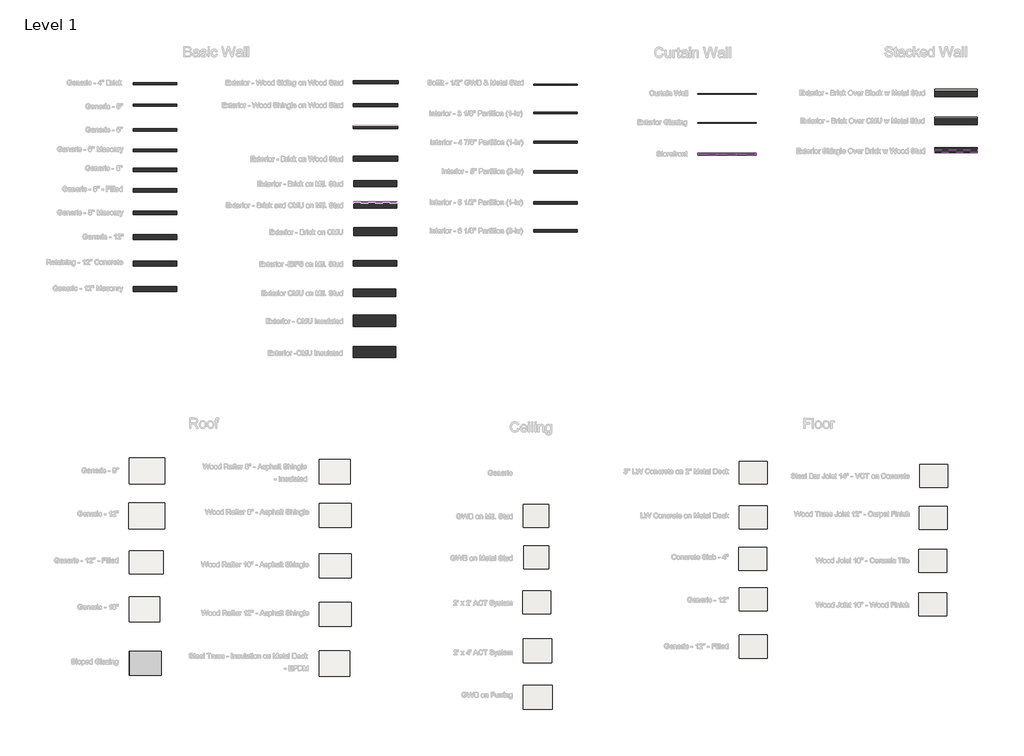
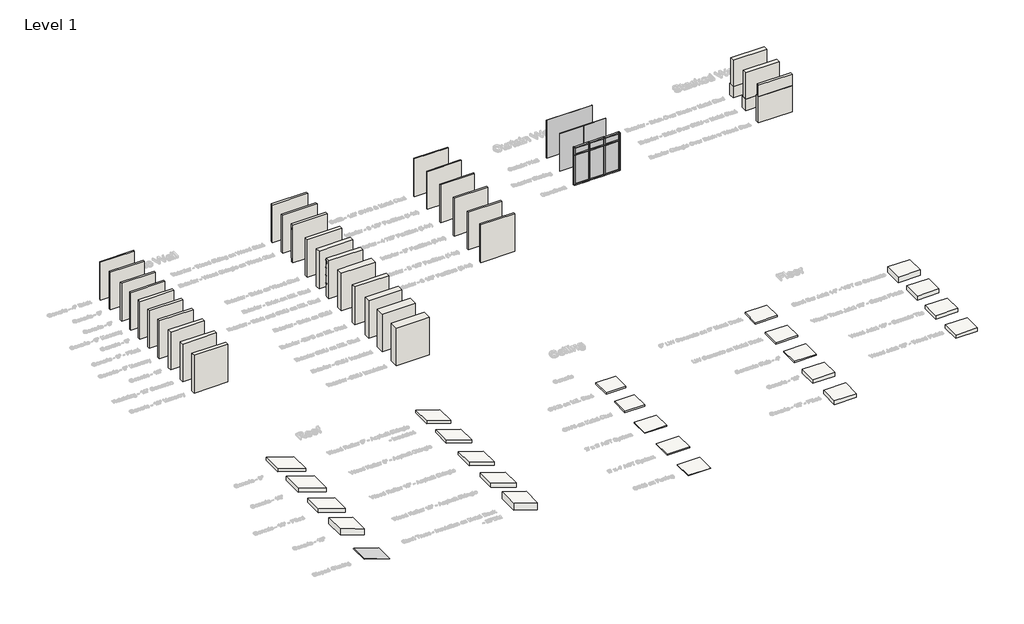
# One storey, part 1 of 42: 33 walls, 17 members, 10 plates, 9 roofs, 9 slabs, 5 coverings, 3 proxies.
"""IFC4 building model written with IfcOpenShell, lengths in millimetres."""

import ifcopenshell
import ifcopenshell.guid

model = None  # the IFC model being written
_history = None  # IfcOwnerHistory: only IFC2X3 demands one
_inside = {}  # id of a spatial element -> (the spatial element, [elements in it])
_under = {}  # id of a project, library or spatial element -> (it, [spatial elements below it])
_declared = {}  # id of a project -> (the project, [libraries it declares])
_typed = {}  # id of a type object -> (the type object, [elements of that type])
_made_of = {}  # id of a material, layer set ... -> (it, [elements and type objects made of it])


def new_model(schema):
    """Start an empty IFC model of exactly this schema.

    Asked for "IFC4X3", IfcOpenShell would pick the latest addendum, in which some entities
    have other attributes; the version numbers below select the first issue.
    IFC2X3 requires an IfcOwnerHistory on every rooted entity: one is made here for all.
    """
    global model, _history
    if schema == "IFC4X3":
        model = ifcopenshell.file(schema_version=(4, 3, 0, 0))
    else:
        model = ifcopenshell.file(schema=schema)
    _inside.clear()
    _under.clear()
    _declared.clear()
    _typed.clear()
    _made_of.clear()
    _history = None
    if model.schema == "IFC2X3":
        org = make("IfcOrganization", Name="unknown")
        user = make(
            "IfcPersonAndOrganization",
            ThePerson=make("IfcPerson", FamilyName="unknown"),
            TheOrganization=org,
        )
        app = make(
            "IfcApplication",
            ApplicationDeveloper=org,
            Version="unknown",
            ApplicationFullName="unknown",
            ApplicationIdentifier="unknown",
        )
        _history = make(
            "IfcOwnerHistory",
            OwningUser=user,
            OwningApplication=app,
            ChangeAction="ADDED",
            CreationDate=0,
        )
    return model


def make(cls, **values):
    """One entity of the class cls with the attributes given. An attribute that is None is left unset."""
    return model.create_entity(
        cls, **{name: value for name, value in values.items() if value is not None}
    )


def rooted(cls, **values):
    """An entity with a GlobalId (a new one), such as an element, a storey or a relation."""
    return make(cls, GlobalId=ifcopenshell.guid.new(), OwnerHistory=_history, **values)


def si_unit(unit_type, name, prefix=None):
    """IfcSIUnit, for example si_unit("LENGTHUNIT", "METRE", prefix="MILLI")."""
    return make("IfcSIUnit", UnitType=unit_type, Prefix=prefix, Name=name)


def assignment(units):
    """IfcUnitAssignment: the units of a project."""
    return None if units is None else make("IfcUnitAssignment", Units=units)


def point(xyz):
    """IfcCartesianPoint."""
    return None if xyz is None else make("IfcCartesianPoint", Coordinates=xyz)


def direction(xyz):
    """IfcDirection."""
    return None if xyz is None else make("IfcDirection", DirectionRatios=xyz)


def frame(location, z_axis=None, x_axis=None):
    """IfcAxis2Placement3D, a coordinate frame: its origin and axes. An axis left out is left unset."""
    return make(
        "IfcAxis2Placement3D",
        Location=point(location),
        Axis=direction(z_axis),
        RefDirection=direction(x_axis),
    )


def origin():
    """The frame at (0, 0, 0) with its axes left unset."""
    return frame((0.0, 0.0, 0.0))


def origin_with_axes():
    """The frame at (0, 0, 0) with the z axis (0, 0, 1) and the x axis (1, 0, 0) written out."""
    return frame((0.0, 0.0, 0.0), z_axis=(0.0, 0.0, 1.0), x_axis=(1.0, 0.0, 0.0))


def place(relative_to, where):
    """IfcLocalPlacement: puts the frame where relative to a parent placement (None: the world)."""
    return make(
        "IfcLocalPlacement", PlacementRelTo=relative_to, RelativePlacement=where
    )


def context(
    kind, dimensions, precision=None, world=None, true_north=None, identifier=None
):
    """IfcGeometricRepresentationContext, for example the 3D "Model" context."""
    return make(
        "IfcGeometricRepresentationContext",
        ContextIdentifier=identifier,
        ContextType=kind,
        CoordinateSpaceDimension=dimensions,
        Precision=precision,
        WorldCoordinateSystem=world,
        TrueNorth=true_north,
    )


def project(units=None, contexts=None):
    """IfcProject with its units and contexts."""
    return rooted(
        "IfcProject",
        Name="project",
        RepresentationContexts=contexts,
        UnitsInContext=assignment(units),
    )


def spatial(cls, under=None, at=None, **own):
    """A site, building, storey or space (cls), placed at a placement, below another one or the project."""
    s = rooted(cls, ObjectPlacement=at, **own)
    if under is not None:
        _under.setdefault(under.id(), (under, []))[1].append(s)
    return s


def polyline(points):
    """IfcPolyline through the points."""
    return make("IfcPolyline", Points=[point(p) for p in points])


def outline(outer, holes=None, kind="AREA"):
    """IfcArbitraryClosedProfileDef: a profile drawn as a closed curve; with holes, ...WithVoids."""
    if holes is None:
        return make("IfcArbitraryClosedProfileDef", ProfileType=kind, OuterCurve=outer)
    return make(
        "IfcArbitraryProfileDefWithVoids",
        ProfileType=kind,
        OuterCurve=outer,
        InnerCurves=holes,
    )


def extrude(swept, where, along, depth):
    """IfcExtrudedAreaSolid: the profile swept, set in the frame where, extruded along a direction by depth."""
    return make(
        "IfcExtrudedAreaSolid",
        SweptArea=swept,
        Position=where,
        ExtrudedDirection=direction(along),
        Depth=depth,
    )


def faces_of(points, faces, orient=None, outer=None):
    """IfcFace entities. A face is a list of loops; a loop is a list of indices into points, from 0.

    orient and outer hold one flag for each loop. By default every Orientation is true, the
    first loop of a face is its IfcFaceOuterBound and the others are IfcFaceBound.
    """
    made = []
    for i, loops in enumerate(faces):
        bounds = []
        for j, loop in enumerate(loops):
            is_outer = j == 0 if outer is None else outer[i][j]
            bounds.append(
                make(
                    "IfcFaceOuterBound" if is_outer else "IfcFaceBound",
                    Bound=make("IfcPolyLoop", Polygon=[points[k] for k in loop]),
                    Orientation=True if orient is None else orient[i][j],
                )
            )
        made.append(make("IfcFace", Bounds=bounds))
    return made


def faceted_brep(points, faces, orient=None, outer=None, voids=None):
    """IfcFacetedBrep: a solid bounded by flat faces; with voids (closed shells), ...WithVoids."""
    shared = [point(p) for p in points]
    hull = make("IfcClosedShell", CfsFaces=faces_of(shared, faces, orient, outer))
    if voids is None:
        return make("IfcFacetedBrep", Outer=hull)
    return make(
        "IfcFacetedBrepWithVoids",
        Outer=hull,
        Voids=[
            make(cls, CfsFaces=faces_of(shared, fs, o, b)) for cls, fs, o, b in voids
        ],
    )


def shape(context_of_items, identifier, shape_type, items):
    """IfcShapeRepresentation: the items that make up one representation, for example the "Body"."""
    return make(
        "IfcShapeRepresentation",
        ContextOfItems=context_of_items,
        RepresentationIdentifier=identifier,
        RepresentationType=shape_type,
        Items=items,
    )


def source(mapping_origin, context_of_items, identifier, shape_type, items):
    """IfcRepresentationMap: a shape defined once, which mapped items show again and again."""
    return make(
        "IfcRepresentationMap",
        MappingOrigin=mapping_origin,
        MappedRepresentation=shape(context_of_items, identifier, shape_type, items),
    )


def transform(
    local_origin,
    x_axis=None,
    y_axis=None,
    z_axis=None,
    scale=None,
    scale2=None,
    scale3=None,
    uniform=True,
):
    """IfcCartesianTransformationOperator3D, or its non-uniform kind. x_axis, y_axis, z_axis: its Axis1, 2, 3."""
    if uniform:
        return make(
            "IfcCartesianTransformationOperator3D",
            Axis1=direction(x_axis),
            Axis2=direction(y_axis),
            LocalOrigin=point(local_origin),
            Scale=scale,
            Axis3=direction(z_axis),
        )
    return make(
        "IfcCartesianTransformationOperator3DnonUniform",
        Axis1=direction(x_axis),
        Axis2=direction(y_axis),
        LocalOrigin=point(local_origin),
        Scale=scale,
        Axis3=direction(z_axis),
        Scale2=scale2,
        Scale3=scale3,
    )


def mapped(mapping_source, mapping_target):
    """IfcMappedItem: shows the shape of a source again, moved by a transform."""
    return make(
        "IfcMappedItem", MappingSource=mapping_source, MappingTarget=mapping_target
    )


def made_of(thing, what):
    """Note that an element or type object is made of a material, layer set ...; save() writes the relation."""
    if what is not None:
        _made_of.setdefault(what.id(), (what, []))[1].append(thing)
    return thing


def element(
    cls,
    number,
    at=None,
    inside=None,
    cuts=None,
    type_object=None,
    material=None,
    context=None,
    identifier="Body",
    shape_type=None,
    held_by="IfcProductDefinitionShape",
    body=None,
    shapes=None,
    **own,
):
    """One element of the class cls, such as IfcWall. Its Tag is "e" and its number.

    at: its placement. inside: the storey or other place that contains it. cuts: it is an
    opening in that element (IfcRelVoidsElement). A single representation is given by context,
    identifier, shape_type and body (its items); several are given by shapes. held_by: the class
    of the entity that holds the representations. save() writes the other relations.
    """
    e = rooted(cls, Tag="e%d" % number, ObjectPlacement=at, **own)
    if body is not None:
        shapes = [shape(context, identifier, shape_type, body)]
    if shapes is not None:
        e.Representation = make(held_by, Representations=shapes)
    if inside is not None:
        _inside.setdefault(inside.id(), (inside, []))[1].append(e)
    if cuts is not None:
        rooted(
            "IfcRelVoidsElement", RelatingBuildingElement=cuts, RelatedOpeningElement=e
        )
    if type_object is not None:
        _typed.setdefault(type_object.id(), (type_object, []))[1].append(e)
    return made_of(e, material)


def aggregate(whole, parts):
    """IfcRelAggregates: a whole, such as a stair, and the parts it consists of."""
    return rooted("IfcRelAggregates", RelatingObject=whole, RelatedObjects=parts)


def save(model, path):
    """Write the relations noted so far, then the file.

    IfcRelAggregates (storeys below a building ...), IfcRelContainedInSpatialStructure (elements
    in a storey), IfcRelDefinesByType, IfcRelAssociatesMaterial and IfcRelDeclares: one each for
    every whole, place, type object, material and project.
    """
    for whole, parts in _under.values():
        aggregate(whole, parts)
    for where, things in _inside.values():
        rooted(
            "IfcRelContainedInSpatialStructure",
            RelatedElements=things,
            RelatingStructure=where,
        )
    for kind, things in _typed.values():
        rooted("IfcRelDefinesByType", RelatedObjects=things, RelatingType=kind)
    for what, things in _made_of.values():
        rooted("IfcRelAssociatesMaterial", RelatedObjects=things, RelatingMaterial=what)
    for by, libraries in _declared.values():
        rooted("IfcRelDeclares", RelatingContext=by, RelatedDefinitions=libraries)
    model.write(path)


def member_f0fea5a5(model_context):
    return source(origin(), model_context, "Body", "SweptSolid", [
        extrude(outline(polyline([(31.75, 63.5), (31.75, -63.5), (-31.75, -63.5), (-31.75, 63.5), (31.75, 63.5)])), frame((0.0, 0.0, -2438.4), z_axis=(0.0, 0.0, 1.0), x_axis=(1.0, 0.0, 0.0)), (0.0, 0.0, 1.0), 2438.4),
    ])


def member_ee409385(model_context):
    return source(origin(), model_context, "Body", "SweptSolid", [
        extrude(outline(polyline([(0.0, 63.5), (0.0, -63.5), (-63.5, -63.5), (-63.5, 63.5), (0.0, 63.5)])), frame((0.0, 0.0, -2438.4), z_axis=(0.0, 0.0, 1.0), x_axis=(1.0, 0.0, 0.0)), (0.0, 0.0, 1.0), 2438.4),
    ])


def member_6e77e263(model_context):
    return source(origin(), model_context, "Body", "SweptSolid", [
        extrude(outline(polyline([(31.75, 63.5), (31.75, -63.5), (-31.75, -63.5), (-31.75, 63.5), (31.75, 63.5)])), frame((0.0, 0.0, -609.6), z_axis=(0.0, 0.0, 1.0), x_axis=(1.0, 0.0, 0.0)), (0.0, 0.0, 1.0), 609.6),
    ])


def member_47bfaf8a(model_context):
    return source(origin(), model_context, "Body", "SweptSolid", [
        extrude(outline(polyline([(0.0, 63.5), (0.0, -63.5), (-63.5, -63.5), (-63.5, 63.5), (0.0, 63.5)])), frame((0.0, 0.0, -609.6), z_axis=(0.0, 0.0, 1.0), x_axis=(1.0, 0.0, 0.0)), (0.0, 0.0, 1.0), 609.6),
    ])


def member_9b1c5889(model_context):
    return source(origin(), model_context, "Body", "SweptSolid", [
        extrude(outline(polyline([(0.0, 63.5), (0.0, -63.5), (-63.5, -63.5), (-63.5, 63.5), (0.0, 63.5)])), frame((0.0, 0.0, -1073.1500001), z_axis=(0.0, 0.0, 1.0), x_axis=(1.0, 0.0, 0.0)), (0.0, 0.0, 1.0), 1073.1500001),
    ])


def member_f5e9651f(model_context):
    return source(origin(), model_context, "Body", "SweptSolid", [
        extrude(outline(polyline([(0.0, 63.5), (0.0, -63.5), (-63.5, -63.5), (-63.5, 63.5), (0.0, 63.5)])), frame((0.0, 0.0, -1104.8999998), z_axis=(0.0, 0.0, 1.0), x_axis=(1.0, 0.0, 0.0)), (0.0, 0.0, 1.0), 1104.8999998),
    ])


def member_0f61b456(model_context):
    return source(origin(), model_context, "Body", "SweptSolid", [
        extrude(outline(polyline([(31.75, 63.5), (31.75, -63.5), (-31.75, -63.5), (-31.75, 63.5), (31.75, 63.5)])), frame((0.0, 0.0, -1073.1500001), z_axis=(0.0, 0.0, 1.0), x_axis=(1.0, 0.0, 0.0)), (0.0, 0.0, 1.0), 1073.1500001),
    ])


def member_766f1680(model_context):
    return source(origin(), model_context, "Body", "SweptSolid", [
        extrude(outline(polyline([(31.75, 63.5), (31.75, -63.5), (-31.75, -63.5), (-31.75, 63.5), (31.75, 63.5)])), frame((0.0, 0.0, -1104.8999998), z_axis=(0.0, 0.0, 1.0), x_axis=(1.0, 0.0, 0.0)), (0.0, 0.0, 1.0), 1104.8999998),
    ])


def system_panel_glazed_bff502fa(model_context):
    return source(origin(), model_context, "Body", "SweptSolid", [
        extrude(outline(polyline([(914.4000002, 19.05), (-914.4000002, 19.05), (-914.4000002, 44.45), (914.4000002, 44.45), (914.4000002, 19.05)])), origin_with_axes(), (0.0, 0.0, 1.0), 3048.0),
    ])


def system_panel_glazed_af99cf8b(model_context):
    return source(origin(), model_context, "Body", "SweptSolid", [
        extrude(outline(polyline([(719.3802866, 19.05), (-719.3802866, 19.05), (-719.3802866, 44.45), (719.3802866, 44.45), (719.3802866, 19.05)])), origin_with_axes(), (0.0, 0.0, 1.0), 2032.8912782),
    ])


def system_panel_glazed_0ae67c42(model_context):
    return source(origin(), model_context, "Body", "SweptSolid", [
        extrude(outline(polyline([(1752.6, 19.05), (-1752.6, 19.05), (-1752.6, 44.45), (1752.6, 44.45), (1752.6, 19.05)])), origin_with_axes(), (0.0, 0.0, 1.0), 3048.0),
    ])


def system_panel_glazed_525848d0(model_context):
    return source(origin(), model_context, "Body", "SweptSolid", [
        extrude(outline(polyline([(838.1999998, 19.05), (-838.1999998, 19.05), (-838.1999998, 44.45), (838.1999998, 44.45), (838.1999998, 19.05)])), origin_with_axes(), (0.0, 0.0, 1.0), 3048.0),
    ])


def system_panel_glazed_2e981f09(model_context):
    return source(origin(), model_context, "Body", "SweptSolid", [
        extrude(outline(polyline([(536.5750001, 19.05), (-536.5750001, 19.05), (-536.5750001, 44.45), (536.5750001, 44.45), (536.5750001, 19.05)])), origin_with_axes(), (0.0, 0.0, 1.0), 2343.15),
    ])


def system_panel_glazed_87980334(model_context):
    return source(origin(), model_context, "Body", "SweptSolid", [
        extrude(outline(polyline([(552.4499999, 19.05), (-552.4499999, 19.05), (-552.4499999, 44.45), (552.4499999, 44.45), (552.4499999, 19.05)])), origin_with_axes(), (0.0, 0.0, 1.0), 2343.15),
    ])


def system_panel_glazed_ed20128f(model_context):
    return source(origin(), model_context, "Body", "SweptSolid", [
        extrude(outline(polyline([(536.5750001, 19.05), (-536.5750001, 19.05), (-536.5750001, 44.45), (536.5750001, 44.45), (536.5750001, 19.05)])), origin_with_axes(), (0.0, 0.0, 1.0), 514.35),
    ])


def system_panel_glazed_d57d3c71(model_context):
    return source(origin(), model_context, "Body", "SweptSolid", [
        extrude(outline(polyline([(552.4499999, 19.05), (-552.4499999, 19.05), (-552.4499999, 44.45), (552.4499999, 44.45), (552.4499999, 19.05)])), origin_with_axes(), (0.0, 0.0, 1.0), 514.35),
    ])


model = new_model("IFC4")

# Units and contexts
model_context = context("Model", 3, world=origin())
ifc_project = project(units=[si_unit("LENGTHUNIT", "METRE", prefix="MILLI")], contexts=[model_context])

# Site, building, storey
site = spatial("IfcSite", under=ifc_project)
building = spatial("IfcBuilding", under=site)
storey = spatial("IfcBuildingStorey", under=building, Name="Level 1", Elevation=0.0)

# Proxies
placement = place(None, origin())
element("IfcBuildingElementProxy", 1, Name="Reveals", at=placement, inside=storey, context=model_context, shape_type="SweptSolid", body=[
    extrude(outline(polyline([(684.9886716, 10254.6257244), (684.9886716, 10346.7007244), (3275.7886716, 10346.7007244), (3275.7886716, 10254.6257244), (684.9886716, 10254.6257244)])), frame((0.0, 0.0, 1625.6), z_axis=(0.0, 0.0, 1.0), x_axis=(1.0, 0.0, 0.0)), (0.0, 0.0, 1.0), 67.7333333),
])
element("IfcBuildingElementProxy", 2, Name="Reveals", at=placement, inside=storey, context=model_context, shape_type="SweptSolid", body=[
    extrude(outline(polyline([(684.9886716, 10254.6257244), (684.9886716, 10346.7007244), (3275.7886716, 10346.7007244), (3275.7886716, 10254.6257244), (684.9886716, 10254.6257244)])), frame((0.0, 0.0, 2235.2), z_axis=(0.0, 0.0, 1.0), x_axis=(1.0, 0.0, 0.0)), (0.0, 0.0, 1.0), 67.7333333),
])
element("IfcBuildingElementProxy", 3, Name="Reveals", at=placement, inside=storey, context=model_context, shape_type="SweptSolid", body=[
    extrude(outline(polyline([(684.9886716, 10254.6257244), (684.9886716, 10346.7007244), (3275.7886716, 10346.7007244), (3275.7886716, 10254.6257244), (684.9886716, 10254.6257244)])), frame((0.0, 0.0, 2844.8), z_axis=(0.0, 0.0, 1.0), x_axis=(1.0, 0.0, 0.0)), (0.0, 0.0, 1.0), 67.7333333),
])

# Coverings
element("IfcCovering", 4, ObjectType="2' x 2' ACT System", at=placement, inside=storey, context=model_context, shape_type="SweptSolid", body=[
    extrude(outline(polyline([(12486.8390819, -13034.2537401), (12486.8390819, -14405.8537401), (10810.4390819, -14405.8537401), (10810.4390819, -13034.2537401), (12486.8390819, -13034.2537401)])), frame((0.0, 0.0, 304.8), z_axis=(0.0, 0.0, 1.0), x_axis=(1.0, 0.0, 0.0)), (0.0, 0.0, 1.0), 57.15),
])
element("IfcCovering", 5, ObjectType="2' x 4' ACT System", at=placement, inside=storey, context=model_context, shape_type="SweptSolid", body=[
    extrude(outline(polyline([(12558.4206915, -15892.7367664), (12558.4206915, -17334.8063753), (10844.136245, -17334.8063753), (10844.136245, -15892.7367664), (12558.4206915, -15892.7367664)])), frame((0.0, 0.0, 304.8), z_axis=(0.0, 0.0, 1.0), x_axis=(1.0, 0.0, 0.0)), (0.0, 0.0, 1.0), 57.15),
])
element("IfcCovering", 6, ObjectType="GWB on Furring", at=placement, inside=storey, context=model_context, shape_type="SweptSolid", body=[
    extrude(outline(polyline([(12572.090991, -18676.3446177), (12572.090991, -20118.4142266), (10857.8065445, -20118.4142266), (10857.8065445, -18676.3446177), (12572.090991, -18676.3446177)])), frame((0.0, 0.0, 304.8), z_axis=(0.0, 0.0, 1.0), x_axis=(1.0, 0.0, 0.0)), (0.0, 0.0, 1.0), 31.75),
])
element("IfcCovering", 7, ObjectType="GWB on Metal Stud", at=placement, inside=storey, context=model_context, shape_type="SweptSolid", body=[
    extrude(outline(polyline([(12388.3840045, -10326.9546667), (12388.3840045, -11698.5546667), (10864.3840045, -11698.5546667), (10864.3840045, -10326.9546667), (12388.3840045, -10326.9546667)])), frame((0.0, 0.0, 304.8), z_axis=(0.0, 0.0, 1.0), x_axis=(1.0, 0.0, 0.0)), (0.0, 0.0, 1.0), 104.775),
])
element("IfcCovering", 8, ObjectType="GWB on Mtl. Stud", at=placement, inside=storey, context=model_context, shape_type="SweptSolid", body=[
    extrude(outline(polyline([(12368.9724668, -7850.547691), (12368.9724668, -9222.147691), (10844.9724668, -9222.147691), (10844.9724668, -7850.547691), (12368.9724668, -7850.547691)])), frame((0.0, 0.0, 304.8), z_axis=(0.0, 0.0, 1.0), x_axis=(1.0, 0.0, 0.0)), (0.0, 0.0, 1.0), 107.95),
])

# Members
member_shape = member_f0fea5a5(model_context)
element("IfcMember", 9, ObjectType="Rectangular Mullion : 2.5\" x 5\" rectangular", at=placement, inside=storey, context=model_context, shape_type="MappedRepresentation", body=[
    mapped(member_shape, transform((22476.9663232, 13175.6086881, 0.0), x_axis=(1.0, 0.0, 0.0), y_axis=(0.0, -1.0, 0.0), z_axis=(0.0, 0.0, -1.0))),
])
element("IfcMember", 10, ObjectType="Rectangular Mullion : 2.5\" x 5\" rectangular", at=placement, inside=storey, context=model_context, shape_type="MappedRepresentation", body=[
    mapped(member_shape, transform((23645.366323, 13175.6086881, 0.0), x_axis=(1.0, 0.0, 0.0), y_axis=(0.0, -1.0, 0.0), z_axis=(0.0, 0.0, -1.0))),
])
member_2_shape = member_ee409385(model_context)
element("IfcMember", 11, ObjectType="Rectangular Mullion : 2.5\" x 5\" rectangular", at=placement, inside=storey, context=model_context, shape_type="MappedRepresentation", body=[
    mapped(member_2_shape, transform((24813.7663231, 13175.6086881, 0.0), x_axis=(1.0, 0.0, 0.0), y_axis=(0.0, -1.0, 0.0), z_axis=(0.0, 0.0, -1.0))),
])
element("IfcMember", 12, ObjectType="Rectangular Mullion : 2.5\" x 5\" rectangular", at=placement, inside=storey, context=model_context, shape_type="MappedRepresentation", body=[
    mapped(member_2_shape, transform((21308.5663231, 13175.6086881, 2438.4), x_axis=(-1.0, 0.0, 0.0), y_axis=(0.0, -1.0, 0.0), z_axis=(0.0, 0.0, 1.0))),
])
member_3_shape = member_6e77e263(model_context)
element("IfcMember", 13, ObjectType="Rectangular Mullion : 2.5\" x 5\" rectangular", at=placement, inside=storey, context=model_context, shape_type="MappedRepresentation", body=[
    mapped(member_3_shape, transform((22476.9663232, 13175.6086881, 2438.4), x_axis=(1.0, 0.0, 0.0), y_axis=(0.0, -1.0, 0.0), z_axis=(0.0, 0.0, -1.0))),
])
element("IfcMember", 14, ObjectType="Rectangular Mullion : 2.5\" x 5\" rectangular", at=placement, inside=storey, context=model_context, shape_type="MappedRepresentation", body=[
    mapped(member_3_shape, transform((23645.366323, 13175.6086881, 2438.4), x_axis=(1.0, 0.0, 0.0), y_axis=(0.0, -1.0, 0.0), z_axis=(0.0, 0.0, -1.0))),
])
member_4_shape = member_47bfaf8a(model_context)
element("IfcMember", 15, ObjectType="Rectangular Mullion : 2.5\" x 5\" rectangular", at=placement, inside=storey, context=model_context, shape_type="MappedRepresentation", body=[
    mapped(member_4_shape, transform((24813.7663231, 13175.6086881, 2438.4), x_axis=(1.0, 0.0, 0.0), y_axis=(0.0, -1.0, 0.0), z_axis=(0.0, 0.0, -1.0))),
])
element("IfcMember", 16, ObjectType="Rectangular Mullion : 2.5\" x 5\" rectangular", at=placement, inside=storey, context=model_context, shape_type="MappedRepresentation", body=[
    mapped(member_4_shape, transform((21308.5663231, 13175.6086881, 3048.0), x_axis=(-1.0, 0.0, 0.0), y_axis=(0.0, -1.0, 0.0), z_axis=(0.0, 0.0, 1.0))),
])
member_5_shape = member_9b1c5889(model_context)
element("IfcMember", 17, ObjectType="Rectangular Mullion : 2.5\" x 5\" rectangular", at=placement, inside=storey, context=model_context, shape_type="MappedRepresentation", body=[
    mapped(member_5_shape, transform((24750.2663231, 13175.6086881, 3048.0), x_axis=(0.0, 0.0, 1.0), y_axis=(0.0, -1.0, 0.0), z_axis=(1.0, 0.0, 0.0))),
])
element("IfcMember", 18, ObjectType="Rectangular Mullion : 2.5\" x 5\" rectangular", at=placement, inside=storey, context=model_context, shape_type="MappedRepresentation", body=[
    mapped(member_5_shape, transform((22445.2163232, 13175.6086881, 3048.0), x_axis=(0.0, 0.0, 1.0), y_axis=(0.0, -1.0, 0.0), z_axis=(1.0, 0.0, 0.0))),
])
element("IfcMember", 19, ObjectType="Rectangular Mullion : 2.5\" x 5\" rectangular", at=placement, inside=storey, context=model_context, shape_type="MappedRepresentation", body=[
    mapped(member_5_shape, transform((21372.0663231, 13175.6086881, 0.0), x_axis=(0.0, 0.0, -1.0), y_axis=(0.0, -1.0, 0.0), z_axis=(-1.0, 0.0, 0.0))),
])
element("IfcMember", 20, ObjectType="Rectangular Mullion : 2.5\" x 5\" rectangular", at=placement, inside=storey, context=model_context, shape_type="MappedRepresentation", body=[
    mapped(member_5_shape, transform((23677.116323, 13175.6086881, 0.0), x_axis=(0.0, 0.0, -1.0), y_axis=(0.0, -1.0, 0.0), z_axis=(-1.0, 0.0, 0.0))),
])
member_6_shape = member_f5e9651f(model_context)
element("IfcMember", 21, ObjectType="Rectangular Mullion : 2.5\" x 5\" rectangular", at=placement, inside=storey, context=model_context, shape_type="MappedRepresentation", body=[
    mapped(member_6_shape, transform((22508.7163232, 13175.6086881, 0.0), x_axis=(0.0, 0.0, -1.0), y_axis=(0.0, -1.0, 0.0), z_axis=(-1.0, 0.0, 0.0))),
])
member_7_shape = member_0f61b456(model_context)
element("IfcMember", 22, ObjectType="Rectangular Mullion : 2.5\" x 5\" rectangular", at=placement, inside=storey, context=model_context, shape_type="MappedRepresentation", body=[
    mapped(member_7_shape, transform((22445.2163232, 13175.6086881, 2438.4), x_axis=(0.0, 0.0, 1.0), y_axis=(0.0, -1.0, 0.0), z_axis=(1.0, 0.0, 0.0))),
])
element("IfcMember", 23, ObjectType="Rectangular Mullion : 2.5\" x 5\" rectangular", at=placement, inside=storey, context=model_context, shape_type="MappedRepresentation", body=[
    mapped(member_7_shape, transform((24750.2663231, 13175.6086881, 2438.4), x_axis=(0.0, 0.0, 1.0), y_axis=(0.0, -1.0, 0.0), z_axis=(1.0, 0.0, 0.0))),
])
member_8_shape = member_766f1680(model_context)
element("IfcMember", 24, ObjectType="Rectangular Mullion : 2.5\" x 5\" rectangular", at=placement, inside=storey, context=model_context, shape_type="MappedRepresentation", body=[
    mapped(member_8_shape, transform((23613.616323, 13175.6086881, 2438.4), x_axis=(0.0, 0.0, 1.0), y_axis=(0.0, -1.0, 0.0), z_axis=(1.0, 0.0, 0.0))),
])
element("IfcMember", 25, ObjectType="Rectangular Mullion : 2.5\" x 5\" rectangular", at=placement, inside=storey, context=model_context, shape_type="MappedRepresentation", body=[
    mapped(member_6_shape, transform((23613.616323, 13175.6086881, 3048.0), x_axis=(0.0, 0.0, 1.0), y_axis=(0.0, -1.0, 0.0), z_axis=(1.0, 0.0, 0.0))),
])

# Plates
system_panel_glazed_shape = system_panel_glazed_bff502fa(model_context)
element("IfcPlate", 26, ObjectType="System Panel : Glazed", at=placement, inside=storey, context=model_context, shape_type="MappedRepresentation", body=[
    mapped(system_panel_glazed_shape, transform((22222.9663232, 15004.4086881, 0.0), x_axis=(1.0, 0.0, 0.0), y_axis=(0.0, 1.0, 0.0), z_axis=(0.0, 0.0, 1.0))),
])
system_panel_glazed_2_shape = system_panel_glazed_af99cf8b(model_context)
element("IfcPlate", 27, ObjectType="System Panel : Glazed", at=placement, inside=storey, context=model_context, shape_type="MappedRepresentation", body=[
    mapped(system_panel_glazed_2_shape, transform((-10836.8268287, -17373.1798963, 0.0), x_axis=(0.0, 1.0, 0.0), y_axis=(-0.3162277660168387, 0.0, -0.9486832980505137), z_axis=(-0.9486832980505137, 0.0, 0.3162277660168387))),
])
system_panel_glazed_3_shape = system_panel_glazed_0ae67c42(model_context)
element("IfcPlate", 28, ObjectType="System Panel : Glazed", at=placement, inside=storey, context=model_context, shape_type="MappedRepresentation", body=[
    mapped(system_panel_glazed_3_shape, transform((23061.1663231, 16757.0086881, 0.0), x_axis=(1.0, 0.0, 0.0), y_axis=(0.0, 1.0, 0.0), z_axis=(0.0, 0.0, 1.0))),
])
system_panel_glazed_4_shape = system_panel_glazed_525848d0(model_context)
element("IfcPlate", 29, ObjectType="System Panel : Glazed", at=placement, inside=storey, context=model_context, shape_type="MappedRepresentation", body=[
    mapped(system_panel_glazed_4_shape, transform((23975.5663232, 15004.4086881, 0.0), x_axis=(1.0, 0.0, 0.0), y_axis=(0.0, 1.0, 0.0), z_axis=(0.0, 0.0, 1.0))),
])
system_panel_glazed_5_shape = system_panel_glazed_2e981f09(model_context)
element("IfcPlate", 30, ObjectType="System Panel : Glazed", at=placement, inside=storey, context=model_context, shape_type="MappedRepresentation", body=[
    mapped(system_panel_glazed_5_shape, transform((21908.6413231, 13175.6086881, 63.5), x_axis=(1.0, 0.0, 0.0), y_axis=(0.0, 1.0, 0.0), z_axis=(0.0, 0.0, 1.0))),
])
element("IfcPlate", 31, ObjectType="System Panel : Glazed", at=placement, inside=storey, context=model_context, shape_type="MappedRepresentation", body=[
    mapped(system_panel_glazed_5_shape, transform((24213.691323, 13175.6086881, 63.5), x_axis=(1.0, 0.0, 0.0), y_axis=(0.0, 1.0, 0.0), z_axis=(0.0, 0.0, 1.0))),
])
system_panel_glazed_6_shape = system_panel_glazed_87980334(model_context)
element("IfcPlate", 32, ObjectType="System Panel : Glazed", at=placement, inside=storey, context=model_context, shape_type="MappedRepresentation", body=[
    mapped(system_panel_glazed_6_shape, transform((23061.1663231, 13175.6086881, 63.5), x_axis=(1.0, 0.0, 0.0), y_axis=(0.0, 1.0, 0.0), z_axis=(0.0, 0.0, 1.0))),
])
system_panel_glazed_7_shape = system_panel_glazed_ed20128f(model_context)
element("IfcPlate", 33, ObjectType="System Panel : Glazed", at=placement, inside=storey, context=model_context, shape_type="MappedRepresentation", body=[
    mapped(system_panel_glazed_7_shape, transform((21908.6413231, 13175.6086881, 2470.15), x_axis=(1.0, 0.0, 0.0), y_axis=(0.0, 1.0, 0.0), z_axis=(0.0, 0.0, 1.0))),
])
element("IfcPlate", 34, ObjectType="System Panel : Glazed", at=placement, inside=storey, context=model_context, shape_type="MappedRepresentation", body=[
    mapped(system_panel_glazed_7_shape, transform((24213.691323, 13175.6086881, 2470.15), x_axis=(1.0, 0.0, 0.0), y_axis=(0.0, 1.0, 0.0), z_axis=(0.0, 0.0, 1.0))),
])
system_panel_glazed_8_shape = system_panel_glazed_d57d3c71(model_context)
element("IfcPlate", 35, ObjectType="System Panel : Glazed", at=placement, inside=storey, context=model_context, shape_type="MappedRepresentation", body=[
    mapped(system_panel_glazed_8_shape, transform((23061.1663231, 13175.6086881, 2470.15), x_axis=(1.0, 0.0, 0.0), y_axis=(0.0, 1.0, 0.0), z_axis=(0.0, 0.0, 1.0))),
])

# Roofs
element("IfcRoof", 36, ObjectType="Generic - 12\"", at=placement, inside=storey, context=model_context, shape_type="SweptSolid", body=[
    extrude(outline(polyline([(321.2874103, -10641.6185973), (1036.789438, -12788.1246804), (715.5020277, -12788.1246804), (0.0, -10641.6185973), (321.2874103, -10641.6185973)])), frame((0.0, -9316.4021182, 0.0), z_axis=(0.0, 1.0, 0.0), x_axis=(0.0, 0.0, 1.0)), (0.0, 0.0, 1.0), 1579.5625),
])
element("IfcRoof", 37, ObjectType="Generic - 12\" - Filled", at=placement, inside=storey, context=model_context, shape_type="SweptSolid", body=[
    extrude(outline(polyline([(321.2874103, -10734.0001224), (1003.1050879, -12779.4531552), (681.8176776, -12779.4531552), (0.0, -10734.0001224), (321.2874103, -10734.0001224)])), frame((0.0, -12001.3744682, 0.0), z_axis=(0.0, 1.0, 0.0), x_axis=(0.0, 0.0, 1.0)), (0.0, 0.0, 1.0), 1383.6280937),
])
element("IfcRoof", 38, ObjectType="Generic - 18\"", at=placement, inside=storey, context=model_context, shape_type="SweptSolid", body=[
    extrude(outline(polyline([(481.9311154, -10928.8051732), (1098.8137761, -12779.4531552), (616.8826607, -12779.4531552), (0.0, -10928.8051732), (481.9311154, -10928.8051732)])), frame((0.0, -14869.9869682, 0.0), z_axis=(0.0, 1.0, 0.0), x_axis=(0.0, 0.0, 1.0)), (0.0, 0.0, 1.0), 1497.2020884),
])
element("IfcRoof", 39, ObjectType="Generic - 9\"", at=placement, inside=storey, context=model_context, shape_type="SweptSolid", body=[
    extrude(outline(polyline([(240.9655577, -10645.8531552), (952.1655577, -12779.4531552), (711.2, -12779.4531552), (0.0, -10645.8531552), (240.9655577, -10645.8531552)])), frame((0.0, -6597.0146182, 0.0), z_axis=(0.0, 1.0, 0.0), x_axis=(0.0, 0.0, 1.0)), (0.0, 0.0, 1.0), 1534.3628563),
])
element("IfcRoof", 40, ObjectType="Steel Truss - Insulation on Metal Deck - EPDM", at=placement, inside=storey, context=model_context, shape_type="SweptSolid", body=[
    extrude(outline(polyline([(575.6399434, 451.8559594), (1185.2399434, -1376.9440406), (609.6, -1376.9440406), (0.0, 451.8559594), (575.6399434, 451.8559594)])), frame((0.0, -18138.4509823, 0.0), z_axis=(0.0, 1.0, 0.0), x_axis=(0.0, 0.0, 1.0)), (0.0, 0.0, 1.0), 1524.0),
])
element("IfcRoof", 41, ObjectType="Wood Rafter 10\" - Asphalt Shingle", at=placement, inside=storey, context=model_context, shape_type="SweptSolid", body=[
    extrude(outline(polyline([(274.4329963, 542.7798174), (917.2896637, -1385.790185), (642.8566675, -1385.790185), (0.0, 542.7798174), (274.4329963, 542.7798174)])), frame((0.0, -12251.6321179, 0.0), z_axis=(0.0, 1.0, 0.0), x_axis=(0.0, 0.0, 1.0)), (0.0, 0.0, 1.0), 1438.7605731),
])
element("IfcRoof", 42, ObjectType="Wood Rafter 12\" - Asphalt Shingle", at=placement, inside=storey, context=model_context, shape_type="SweptSolid", body=[
    extrude(outline(polyline([(327.980898, 542.7798174), (970.8375654, -1385.790185), (642.8566675, -1385.790185), (0.0, 542.7798174), (327.980898, 542.7798174)])), frame((0.0, -15148.992691, 0.0), z_axis=(0.0, 1.0, 0.0), x_axis=(0.0, 0.0, 1.0)), (0.0, 0.0, 1.0), 1438.7605731),
])
element("IfcRoof", 43, ObjectType="Wood Rafter 8\" - Asphalt Shingle", at=placement, inside=storey, context=model_context, shape_type="SweptSolid", body=[
    extrude(outline(polyline([(220.8850946, 545.7910112), (863.741762, -1382.7789912), (642.8566675, -1382.7789912), (0.0, 545.7910112), (220.8850946, 545.7910112)])), frame((0.0, -9229.8693805, 0.0), z_axis=(0.0, 1.0, 0.0), x_axis=(0.0, 0.0, 1.0)), (0.0, 0.0, 1.0), 1438.7605731),
])
element("IfcRoof", 44, ObjectType="Wood Rafter 8\" - Asphalt Shingle - Insulated", at=placement, inside=storey, context=model_context, shape_type="SweptSolid", body=[
    extrude(outline(polyline([(224.2318384, 475.5814538), (841.1144991, -1375.0665283), (616.8826607, -1375.0665283), (0.0, 475.5814538), (224.2318384, 475.5814538)])), frame((0.0, -6594.6223043, 0.0), z_axis=(0.0, 1.0, 0.0), x_axis=(0.0, 0.0, 1.0)), (0.0, 0.0, 1.0), 1445.5405937),
])

# Slabs
element("IfcSlab", 45, ObjectType="Wood Truss  Joist 12\" - Carpet Finish ", at=placement, inside=storey, context=model_context, shape_type="SweptSolid", body=[
    extrude(outline(polyline([(36266.767036, -7964.1153855), (36266.767036, -9335.7153855), (34590.367036, -9335.7153855), (34590.367036, -7964.1153855), (36266.767036, -7964.1153855)])), frame((0.0, 0.0, -323.85), z_axis=(0.0, 0.0, 1.0), x_axis=(1.0, 0.0, 0.0)), (0.0, 0.0, 1.0), 323.85),
])
element("IfcSlab", 46, ObjectType="3\" LW Concrete on 2\" Metal Deck", at=placement, inside=storey, context=model_context, shape_type="SweptSolid", body=[
    extrude(outline(polyline([(25462.297259, -5250.8171932), (25462.297259, -6622.4171932), (23785.897259, -6622.4171932), (23785.897259, -5250.8171932), (25462.297259, -5250.8171932)])), frame((0.0, 0.0, -127.0), z_axis=(0.0, 0.0, 1.0), x_axis=(1.0, 0.0, 0.0)), (0.0, 0.0, 1.0), 127.0),
])
element("IfcSlab", 47, ObjectType="Concrete Slab - 4\"", at=placement, inside=storey, context=model_context, shape_type="SweptSolid", body=[
    extrude(outline(polyline([(25449.5750317, -10417.8079652), (25449.5750317, -11789.4079652), (23773.1750317, -11789.4079652), (23773.1750317, -10417.8079652), (25449.5750317, -10417.8079652)])), frame((0.0, 0.0, -101.6), z_axis=(0.0, 0.0, 1.0), x_axis=(1.0, 0.0, 0.0)), (0.0, 0.0, 1.0), 101.6),
])
element("IfcSlab", 48, ObjectType="Generic - 12\"", at=placement, inside=storey, context=model_context, shape_type="SweptSolid", body=[
    extrude(outline(polyline([(25457.124359, -12846.3368689), (25457.124359, -14217.9368689), (23780.724359, -14217.9368689), (23780.724359, -12846.3368689), (25457.124359, -12846.3368689)])), frame((0.0, 0.0, -304.8), z_axis=(0.0, 0.0, 1.0), x_axis=(1.0, 0.0, 0.0)), (0.0, 0.0, 1.0), 304.8),
])
element("IfcSlab", 49, ObjectType="Generic - 12\" - Filled", at=placement, inside=storey, context=model_context, shape_type="SweptSolid", body=[
    extrude(outline(polyline([(25473.8528339, -15648.3022704), (25473.8528339, -17070.7022704), (23797.4528339, -17070.7022704), (23797.4528339, -15648.3022704), (25473.8528339, -15648.3022704)])), frame((0.0, 0.0, -304.8), z_axis=(0.0, 0.0, 1.0), x_axis=(1.0, 0.0, 0.0)), (0.0, 0.0, 1.0), 304.8),
])
element("IfcSlab", 50, ObjectType="LW Concrete on Metal Deck", at=placement, inside=storey, context=model_context, shape_type="SweptSolid", body=[
    extrude(outline(polyline([(25464.6636445, -7938.3779014), (25464.6636445, -9309.9779014), (23788.2636445, -9309.9779014), (23788.2636445, -7938.3779014), (25464.6636445, -7938.3779014)])), frame((0.0, 0.0, -104.775), z_axis=(0.0, 0.0, 1.0), x_axis=(1.0, 0.0, 0.0)), (0.0, 0.0, 1.0), 104.775),
])
element("IfcSlab", 51, ObjectType="Steel Bar Joist 14\" - VCT on Concrete", at=placement, inside=storey, context=model_context, shape_type="SweptSolid", body=[
    extrude(outline(polyline([(36284.0122585, -5434.5515682), (36284.0122585, -6806.1515682), (34607.6122585, -6806.1515682), (34607.6122585, -5434.5515682), (36284.0122585, -5434.5515682)])), frame((0.0, 0.0, -441.325), z_axis=(0.0, 0.0, 1.0), x_axis=(1.0, 0.0, 0.0)), (0.0, 0.0, 1.0), 441.325),
])
element("IfcSlab", 52, ObjectType="Wood Joist 10\" - Ceramic Tile", at=placement, inside=storey, context=model_context, shape_type="SweptSolid", body=[
    extrude(outline(polyline([(36216.4995459, -10528.7510967), (36216.4995459, -11900.3510967), (34540.0995459, -11900.3510967), (34540.0995459, -10528.7510967), (36216.4995459, -10528.7510967)])), frame((0.0, 0.0, -273.05), z_axis=(0.0, 0.0, 1.0), x_axis=(1.0, 0.0, 0.0)), (0.0, 0.0, 1.0), 273.05),
])
element("IfcSlab", 53, ObjectType="Wood Joist 10\" - Wood Finish", at=placement, inside=storey, context=model_context, shape_type="SweptSolid", body=[
    extrude(outline(polyline([(36231.4850833, -13137.5746207), (36231.4850833, -14509.1746207), (34555.0850833, -14509.1746207), (34555.0850833, -13137.5746207), (36231.4850833, -13137.5746207)])), frame((0.0, 0.0, -273.05), z_axis=(0.0, 0.0, 1.0), x_axis=(1.0, 0.0, 0.0)), (0.0, 0.0, 1.0), 273.05),
])

# Walls
element("IfcWall", 54, ObjectType="Soffit - 1/2\" GWB & Metal Stud", at=placement, inside=storey, context=model_context, shape_type="SweptSolid", body=[
    extrude(outline(polyline([(14079.2439264, 17311.8960361), (11488.4439264, 17311.8960361), (11488.4439264, 17362.6960361), (14079.2439264, 17362.6960361), (14079.2439264, 17311.8960361)])), origin_with_axes(), (0.0, 0.0, 1.0), 3048.0),
])
element("IfcWall", 55, ObjectType="Exterior - Wood Shingle over Wood Siding on Wood Stud", at=placement, inside=storey, context=model_context, shape_type="Brep", body=[
    faceted_brep([(668.8686716, 14685.8878373, 0.0), (3310.4686716, 14685.8878373, 0.0), (3310.4686716, 14685.8878373, 3048.0), (668.8686716, 14685.8878373, 3048.0), (668.8686716, 14873.2128373, 0.0), (668.8686716, 14873.2128373, 254.0), (668.8686716, 14873.2128373, 2559.05), (668.8686716, 14873.2128373, 2743.2), (668.8686716, 14873.2128373, 3048.0), (3310.4686716, 14873.2128373, 3048.0), (3310.4686716, 14873.2128373, 2743.2), (3310.4686716, 14873.2128373, 2559.05), (3310.4686716, 14873.2128373, 254.0), (3310.4686716, 14873.2128373, 0.0)], [[[0, 1, 2, 3]], [[4, 5, 6, 7, 8, 9, 10, 11, 12, 13]], [[1, 0, 4, 13]], [[2, 1, 13, 12, 11, 10, 9]], [[3, 2, 9, 8]], [[0, 3, 8, 7, 6, 5, 4]]]),
])
element("IfcWall", 56, ObjectType="Exterior - Block on Mtl. Stud", at=placement, inside=storey, context=model_context, shape_type="Brep", body=[
    faceted_brep([(35496.1518113, 16604.091373, 0.0), (38067.522891, 16604.091373, 0.0), (38067.522891, 16604.091373, 900.0), (35496.1518113, 16604.091373, 900.0), (35496.1518113, 17064.091373, 0.0), (35496.1518113, 17064.091373, 900.0), (38067.522891, 17064.091373, 900.0), (38067.522891, 17064.091373, 0.0), (38067.522891, 16956.616373, 900.0), (35496.1518113, 16956.616373, 900.0)], [[[0, 1, 2, 3]], [[4, 5, 6, 7]], [[1, 0, 4, 7]], [[2, 1, 7, 6, 8]], [[3, 2, 8, 6, 5, 9]], [[0, 3, 9, 5, 4]]]),
])
element("IfcWall", 57, ObjectType="Exterior - Brick and CMU on MTL. Stud", at=placement, inside=storey, context=model_context, shape_type="SweptSolid", body=[
    extrude(outline(polyline([(9927.6007244, 0.0), (9927.6007244, 3048.0), (10280.0257244, 3048.0), (10280.0257244, 2912.5333333), (10254.6257244, 2912.5333333), (10254.6257244, 2844.8), (10187.9507244, 2844.8), (10187.9507244, 2641.6), (10280.0257244, 2641.6), (10280.0257244, 2302.9333333), (10254.6257244, 2302.9333333), (10254.6257244, 2235.2), (10280.0257244, 2235.2), (10280.0257244, 1693.3333333), (10254.6257244, 1693.3333333), (10254.6257244, 1625.6), (10280.0257244, 1625.6), (10280.0257244, 1085.85), (10187.9507244, 1085.85), (10187.9507244, 1016.0), (10280.0257244, 1016.0), (10280.0257244, 0.0), (10187.9507244, 0.0), (9927.6007244, 0.0)])), frame((684.9886716, 0.0, 0.0), z_axis=(1.0, 0.0, 0.0), x_axis=(0.0, 1.0, 0.0)), (0.0, 0.0, 1.0), 2590.8),
])
element("IfcWall", 58, ObjectType="Exterior - Brick on CMU", at=placement, inside=storey, context=model_context, shape_type="SweptSolid", body=[
    extrude(outline(polyline([(3275.7886716, 8281.3632244), (684.9886716, 8281.3632244), (684.9886716, 8776.6632244), (3275.7886716, 8776.6632244), (3275.7886716, 8281.3632244)])), origin_with_axes(), (0.0, 0.0, 1.0), 3048.0),
])
element("IfcWall", 59, ObjectType="Exterior - Brick on Mtl. Stud", at=placement, inside=storey, context=model_context, shape_type="SweptSolid", body=[
    extrude(outline(polyline([(3275.7886716, 11223.0007244), (684.9886716, 11223.0007244), (684.9886716, 11575.4257244), (3275.7886716, 11575.4257244), (3275.7886716, 11223.0007244)])), origin_with_axes(), (0.0, 0.0, 1.0), 3048.0),
])
element("IfcWall", 60, ObjectType="Exterior - Brick on Mtl. Stud", at=placement, inside=storey, context=model_context, shape_type="SweptSolid", body=[
    extrude(outline(polyline([(38067.522891, 16604.191373), (35496.1518113, 16604.191373), (35496.1518113, 16956.616373), (38067.522891, 16956.616373), (38067.522891, 16604.191373)])), frame((0.0, 0.0, 900.0), z_axis=(0.0, 0.0, 1.0), x_axis=(1.0, 0.0, 0.0)), (0.0, 0.0, 1.0), 2148.0),
])
element("IfcWall", 61, ObjectType="Exterior - Brick on Mtl. Stud", at=placement, inside=storey, context=model_context, shape_type="SweptSolid", body=[
    extrude(outline(polyline([(38067.522891, 14930.678873), (35496.1518113, 14930.678873), (35496.1518113, 15283.103873), (38067.522891, 15283.103873), (38067.522891, 14930.678873)])), frame((0.0, 0.0, 914.4), z_axis=(0.0, 0.0, 1.0), x_axis=(1.0, 0.0, 0.0)), (0.0, 0.0, 1.0), 2133.6),
])
element("IfcWall", 62, ObjectType="Exterior - Brick on Wood Stud", at=placement, inside=storey, context=model_context, shape_type="SweptSolid", body=[
    extrude(outline(polyline([(3310.4686716, 12758.6628373), (668.8686716, 12758.6628373), (668.8686716, 13041.2378373), (3310.4686716, 13041.2378373), (3310.4686716, 12758.6628373)])), origin_with_axes(), (0.0, 0.0, 1.0), 3048.0),
])
element("IfcWall", 63, ObjectType="Exterior - Brick on Wood Stud", at=placement, inside=storey, context=model_context, shape_type="Brep", body=[
    faceted_brep([(35496.1518113, 13263.803873, 0.0), (38067.522891, 13263.803873, 0.0), (38067.522891, 13263.803873, 2133.6), (35496.1518113, 13263.803873, 2133.6), (35496.1518113, 13546.378873, 0.0), (35496.1518113, 13546.378873, 2133.6), (38067.522891, 13546.378873, 2133.6), (38067.522891, 13546.378873, 0.0), (38067.522891, 13444.778873, 2133.6), (35496.1518113, 13444.778873, 2133.6)], [[[0, 1, 2, 3]], [[4, 5, 6, 7]], [[1, 0, 4, 7]], [[2, 1, 7, 6, 8]], [[3, 2, 8, 6, 5, 9]], [[0, 3, 9, 5, 4]]]),
])
element("IfcWall", 64, ObjectType="Exterior - CMU Insulated", at=placement, inside=storey, context=model_context, shape_type="SweptSolid", body=[
    extrude(outline(polyline([(3205.5597513, 958.2654873), (668.8686716, 958.2654873), (668.8686716, 1631.3654873), (3205.5597513, 1631.3654873), (3205.5597513, 958.2654873)])), origin_with_axes(), (0.0, 0.0, 1.0), 3048.0),
])
element("IfcWall", 65, ObjectType="Exterior - CMU Insulated", at=placement, inside=storey, context=model_context, shape_type="SweptSolid", body=[
    extrude(outline(polyline([(3205.5597513, 2838.5798121), (668.8686716, 2838.5798121), (668.8686716, 3511.6798121), (3205.5597513, 3511.6798121), (3205.5597513, 2838.5798121)])), origin_with_axes(), (0.0, 0.0, 1.0), 3048.0),
])
element("IfcWall", 66, ObjectType="Exterior - CMU on Mtl. Stud", at=placement, inside=storey, context=model_context, shape_type="SweptSolid", body=[
    extrude(outline(polyline([(3205.5597513, 4623.8029873), (668.8686716, 4623.8029873), (668.8686716, 5077.8279873), (3205.5597513, 5077.8279873), (3205.5597513, 4623.8029873)])), origin_with_axes(), (0.0, 0.0, 1.0), 3048.0),
])
element("IfcWall", 67, ObjectType="Exterior - CMU on Mtl. Stud", at=placement, inside=storey, context=model_context, shape_type="Brep", body=[
    faceted_brep([(35496.1518113, 14930.678873, 0.0), (38067.522891, 14930.678873, 0.0), (38067.522891, 14930.678873, 914.4), (35496.1518113, 14930.678873, 914.4), (35496.1518113, 15384.703873, 0.0), (35496.1518113, 15384.703873, 914.4), (38067.522891, 15384.703873, 914.4), (38067.522891, 15384.703873, 0.0), (38067.522891, 15283.103873, 914.4), (35496.1518113, 15283.103873, 914.4)], [[[0, 1, 2, 3]], [[4, 5, 6, 7]], [[1, 0, 4, 7]], [[2, 1, 7, 6, 8]], [[3, 2, 8, 6, 5, 9]], [[0, 3, 9, 5, 4]]]),
])
element("IfcWall", 68, ObjectType="Exterior - EIFS on Mtl. Stud", at=placement, inside=storey, context=model_context, shape_type="SweptSolid", body=[
    extrude(outline(polyline([(3256.3597513, 6466.4963996), (665.5597513, 6466.4963996), (665.5597513, 6777.6463996), (3256.3597513, 6777.6463996), (3256.3597513, 6466.4963996)])), origin_with_axes(), (0.0, 0.0, 1.0), 3048.0),
])
element("IfcWall", 69, ObjectType="Exterior - Wood Shingle on Wood Stud", at=placement, inside=storey, context=model_context, shape_type="SweptSolid", body=[
    extrude(outline(polyline([(3310.4686716, 16011.6548121), (668.8686716, 16011.6548121), (668.8686716, 16192.6298121), (3310.4686716, 16192.6298121), (3310.4686716, 16011.6548121)])), origin_with_axes(), (0.0, 0.0, 1.0), 3048.0),
])
element("IfcWall", 70, ObjectType="Exterior - Wood Shingle on Wood Stud", at=placement, inside=storey, context=model_context, shape_type="SweptSolid", body=[
    extrude(outline(polyline([(38067.522891, 13263.803873), (35496.1518113, 13263.803873), (35496.1518113, 13444.778873), (38067.522891, 13444.778873), (38067.522891, 13263.803873)])), frame((0.0, 0.0, 2133.6), z_axis=(0.0, 0.0, 1.0), x_axis=(1.0, 0.0, 0.0)), (0.0, 0.0, 1.0), 914.4),
])
element("IfcWall", 71, ObjectType="Exterior - Wood Siding on Wood Stud", at=placement, inside=storey, context=model_context, shape_type="SweptSolid", body=[
    extrude(outline(polyline([(3361.2686716, 17381.6673121), (668.8686716, 17381.6673121), (668.8686716, 17565.8173121), (3361.2686716, 17565.8173121), (3361.2686716, 17381.6673121)])), origin_with_axes(), (0.0, 0.0, 1.0), 3048.0),
])
element("IfcWall", 72, ObjectType="Generic - 12\"", at=placement, inside=storey, context=model_context, shape_type="SweptSolid", body=[
    extrude(outline(polyline([(-9931.0043624, 8042.8595608), (-12521.8043624, 8042.8595608), (-12521.8043624, 8347.6595608), (-9931.0043624, 8347.6595608), (-9931.0043624, 8042.8595608)])), origin_with_axes(), (0.0, 0.0, 1.0), 3048.0),
])
element("IfcWall", 73, ObjectType="Generic - 12\" Masonry", at=placement, inside=storey, context=model_context, shape_type="SweptSolid", body=[
    extrude(outline(polyline([(-9931.0043624, 4930.9993236), (-12521.8043624, 4930.9993236), (-12521.8043624, 5226.2743236), (-9931.0043624, 5226.2743236), (-9931.0043624, 4930.9993236)])), origin_with_axes(), (0.0, 0.0, 1.0), 3048.0),
])
element("IfcWall", 74, ObjectType="Generic - 4\" Brick", at=placement, inside=storey, context=model_context, shape_type="SweptSolid", body=[
    extrude(outline(polyline([(-9931.0043624, 17345.7591737), (-12521.8043624, 17345.7591737), (-12521.8043624, 17447.3591737), (-9931.0043624, 17447.3591737), (-9931.0043624, 17345.7591737)])), origin_with_axes(), (0.0, 0.0, 1.0), 3048.0),
])
element("IfcWall", 75, ObjectType="Generic - 5\"", at=placement, inside=storey, context=model_context, shape_type="SweptSolid", body=[
    extrude(outline(polyline([(-9931.0043624, 16037.6591737), (-12521.8043624, 16037.6591737), (-12521.8043624, 16164.6591737), (-9931.0043624, 16164.6591737), (-9931.0043624, 16037.6591737)])), origin_with_axes(), (0.0, 0.0, 1.0), 3048.0),
])
element("IfcWall", 76, ObjectType="Generic - 6\"", at=placement, inside=storey, context=model_context, shape_type="SweptSolid", body=[
    extrude(outline(polyline([(-9931.0043624, 14551.7591737), (-12521.8043624, 14551.7591737), (-12521.8043624, 14704.1591737), (-9931.0043624, 14704.1591737), (-9931.0043624, 14551.7591737)])), origin_with_axes(), (0.0, 0.0, 1.0), 3048.0),
])
element("IfcWall", 77, ObjectType="Generic - 6\" Masonry", at=placement, inside=storey, context=model_context, shape_type="SweptSolid", body=[
    extrude(outline(polyline([(-9931.0043624, 13311.9216737), (-12521.8043624, 13311.9216737), (-12521.8043624, 13454.7966737), (-9931.0043624, 13454.7966737), (-9931.0043624, 13311.9216737)])), origin_with_axes(), (0.0, 0.0, 1.0), 3048.0),
])
element("IfcWall", 78, ObjectType="Generic - 8\"", at=placement, inside=storey, context=model_context, shape_type="SweptSolid", body=[
    extrude(outline(polyline([(-9931.0043624, 12130.770889), (-12521.8043624, 12130.770889), (-12521.8043624, 12333.970889), (-9931.0043624, 12333.970889), (-9931.0043624, 12130.770889)])), origin_with_axes(), (0.0, 0.0, 1.0), 3048.0),
])
element("IfcWall", 79, ObjectType="Generic - 8\" - Filled", at=placement, inside=storey, context=model_context, shape_type="SweptSolid", body=[
    extrude(outline(polyline([(-9931.0043624, 10887.5688588), (-12521.8043624, 10887.5688588), (-12521.8043624, 11090.7688588), (-9931.0043624, 11090.7688588), (-9931.0043624, 10887.5688588)])), origin_with_axes(), (0.0, 0.0, 1.0), 3048.0),
])
element("IfcWall", 80, ObjectType="Generic - 8\" Masonry", at=placement, inside=storey, context=model_context, shape_type="SweptSolid", body=[
    extrude(outline(polyline([(-9931.0043624, 9546.2220608), (-12521.8043624, 9546.2220608), (-12521.8043624, 9739.8970608), (-9931.0043624, 9739.8970608), (-9931.0043624, 9546.2220608)])), origin_with_axes(), (0.0, 0.0, 1.0), 3048.0),
])
element("IfcWall", 81, ObjectType="Interior - 3 1/8\" Partition (1-hr)", at=placement, inside=storey, context=model_context, shape_type="SweptSolid", body=[
    extrude(outline(polyline([(14079.2439264, 15595.8085361), (11488.4439264, 15595.8085361), (11488.4439264, 15675.1835361), (14079.2439264, 15675.1835361), (14079.2439264, 15595.8085361)])), origin_with_axes(), (0.0, 0.0, 1.0), 3048.0),
])
element("IfcWall", 82, ObjectType="Interior - 4 7/8\" Partition (1-hr)", at=placement, inside=storey, context=model_context, shape_type="SweptSolid", body=[
    extrude(outline(polyline([(14079.2439264, 13820.9835361), (11488.4439264, 13820.9835361), (11488.4439264, 13944.8085361), (14079.2439264, 13944.8085361), (14079.2439264, 13820.9835361)])), origin_with_axes(), (0.0, 0.0, 1.0), 3048.0),
])
element("IfcWall", 83, ObjectType="Interior - 5 1/2\" Partition (1-hr)", at=placement, inside=storey, context=model_context, shape_type="SweptSolid", body=[
    extrude(outline(polyline([(14079.2439264, 10177.7661485), (11488.4439264, 10177.7661485), (11488.4439264, 10317.4661485), (14079.2439264, 10317.4661485), (14079.2439264, 10177.7661485)])), origin_with_axes(), (0.0, 0.0, 1.0), 3048.0),
])
element("IfcWall", 84, ObjectType="Interior - 5\" Partition (2-hr)", at=placement, inside=storey, context=model_context, shape_type="SweptSolid", body=[
    extrude(outline(polyline([(14079.2439264, 12038.3161485), (11488.4439264, 12038.3161485), (11488.4439264, 12165.3161485), (14079.2439264, 12165.3161485), (14079.2439264, 12038.3161485)])), origin_with_axes(), (0.0, 0.0, 1.0), 3048.0),
])
element("IfcWall", 85, ObjectType="Interior - 6 1/8\" Partition (2-hr)", at=placement, inside=storey, context=model_context, shape_type="SweptSolid", body=[
    extrude(outline(polyline([(14079.2439264, 8487.7382244), (11488.4439264, 8487.7382244), (11488.4439264, 8643.3132244), (14079.2439264, 8643.3132244), (14079.2439264, 8487.7382244)])), origin_with_axes(), (0.0, 0.0, 1.0), 3048.0),
])
element("IfcWall", 86, ObjectType="Retaining - 12\" Concrete", at=placement, inside=storey, context=model_context, shape_type="SweptSolid", body=[
    extrude(outline(polyline([(-9931.0043624, 6450.2368236), (-12521.8043624, 6450.2368236), (-12521.8043624, 6755.0368236), (-9931.0043624, 6755.0368236), (-9931.0043624, 6450.2368236)])), origin_with_axes(), (0.0, 0.0, 1.0), 3048.0),
])

save(model, "model.ifc")

# Revit data of these elements
# Project information
#   Project Issue Date = "Issue Date"
#   Project Status = "Project Status"
#   Client Name = "Owner"
#   Project Address = "Enter address here"
#   Project Name = "Project Name"
#   Project Number = "Project Number"
# Type "2' x 2' ACT System"
#   Assembly Code = "C3030210"
#   built-in parameter 1002203 = 1 (stored number, unit not read)
#   built-in parameter 1002202 = 1 (stored number, unit not read)
#   Layers, outside or top first: 0' - 1 5/8" "Default" (function 1); 0' - 0 5/8" "Acoustic Ceiling Tile 24 x 24" (function 5)
# Type "2' x 4' ACT System"
#   Assembly Code = "C3030210"
#   built-in parameter 1002203 = 1 (stored number, unit not read)
#   built-in parameter 1002202 = 1 (stored number, unit not read)
#   Layers, outside or top first: 0' - 1 5/8" "Default" (function 1); 0' - 0 5/8" "Acoustic Ceiling Tile 24 x 48" (function 5)
# Type "GWB on Furring"
#   Assembly Code = "C3030220"
#   built-in parameter 1002203 = 1 (stored number, unit not read)
#   built-in parameter 1002202 = 1 (stored number, unit not read)
#   Layers, outside or top first: 0' - 0 3/4" "Metal Stud Layer" (function 1); 0' - 0 1/2" "Gypsum Wall Board" (function 5)
# Type "GWB on Metal Stud"
#   Assembly Code = "C3030220"
#   built-in parameter 1002203 = 1 (stored number, unit not read)
#   built-in parameter 1002202 = 1 (stored number, unit not read)
#   Layers, outside or top first: 0' - 3 5/8" "Metal Stud Layer" (function 1); 0' - 0 1/2" "Gypsum Wall Board" (function 5)
# Type "GWB on Mtl. Stud"
#   Assembly Code = "C3030220"
#   built-in parameter 1002203 = 1 (stored number, unit not read)
#   built-in parameter 1002202 = 1 (stored number, unit not read)
#   Layers, outside or top first: 0' - 3 5/8" "Metal Stud Layer" (function 1); 0' - 0 5/8" "Gypsum Wall Board" (function 5)
# Type "Rectangular Mullion : 2.5\" x 5\" rectangular"
#   built-in parameter 1007304 = 0.416667 (stored number, unit not read)
#   built-in parameter 1007301 = 0.104167 (stored number, unit not read)
#   built-in parameter 1007300 = 0.104167 (stored number, unit not read)
# Type "System Panel : Glazed"
#   Construction Type Id = "GSP4R"
#   Analytic Construction = "1/8 in Pilkington single glazing"
#   Visual Light Transmittance = 0.9
#   Solar Heat Gain Coefficient = 0.86
#   Heat Transfer Coefficient (U) = 1.18115 BTU/(h·ft²·°F)
#   Define Thermal Properties by = 1
# Type "Generic - 12\""
#   Assembly Code = "B1020"
#   Layers, outside or top first: 1' - 0" no material (function 1)
# Type "Generic - 12\" - Filled"
#   Assembly Code = "B1020"
#   Layers, outside or top first: 1' - 0" no material (function 1)
# Type "Generic - 18\""
#   Assembly Code = "B1020"
#   Layers, outside or top first: 1' - 6" no material (function 1)
# Type "Generic - 9\""
#   Assembly Code = "B1020"
#   Layers, outside or top first: 0' - 9" no material (function 1)
# Type "Steel Truss - Insulation on Metal Deck - EPDM"
#   Assembly Code = "B1020"
#   Layers, outside or top first: 0' - 0 1/4" "Roofing, EPDM Membrane" (function 4); 0' - 5" "Rigid insulation" (function 3); 0' - 0 1/4" "Metal Deck" (function 1); 1' - 4" "Structure, Steel Bar Joist Layer" (function 1)
# Type "Wood Rafter 10\" - Asphalt Shingle"
#   Assembly Code = "B1020"
#   Layers, outside or top first: 0' - 0 1/4" "Asphalt Shingle" (function 4); 0' - 0 3/4" "Plywood, Sheathing" (function 2); 0' - 9 1/4" "Structure, Wood Joist/Rafter Layer, Batt Insulation" (function 1)
# Type "Wood Rafter 12\" - Asphalt Shingle"
#   Assembly Code = "B1020"
#   Layers, outside or top first: 0' - 0 1/4" "Asphalt Shingle" (function 4); 0' - 0 3/4" "Plywood, Sheathing" (function 2); 0' - 11 1/4" "Structure, Wood Joist/Rafter Layer, Batt Insulation" (function 1)
# Type "Wood Rafter 8\" - Asphalt Shingle"
#   Assembly Code = "B1020"
#   Layers, outside or top first: 0' - 0 1/4" "Asphalt Shingle" (function 4); 0' - 0 3/4" "Plywood, Sheathing" (function 2); 0' - 7 1/4" "Structure, Wood Joist/Rafter Layer, Batt Insulation" (function 1)
# Type "Wood Rafter 8\" - Asphalt Shingle - Insulated"
#   Assembly Code = "B1020"
#   Layers, outside or top first: 0' - 0 1/4" "Asphalt Shingle" (function 4); 0' - 0 5/8" "Plywood, Sheathing" (function 2); 0' - 7 1/2" "Structure, Wood Joist/Rafter Layer, Batt Insulation" (function 1)
# Type "Wood Truss  Joist 12\" - Carpet Finish "
#   Assembly Code = "B1010"
#   Function = 0
#   Layers, outside or top first: 0' - 0 1/8" "Carpet (1)" (function 4); 0' - 0 3/4" "Plywood, Sheathing" (function 1); 0' - 11 7/8" "Structure, Wood Joist/Rafter Layer" (function 1)
# Type "3\" LW Concrete on 2\" Metal Deck"
#   Assembly Code = "B1010"
#   Function = 0
#   Layers, outside or top first: 0' - 5" "Concrete, Lightweight" (function 1); 0' - 0" "Metal Deck" (function 200)
# Type "Concrete Slab - 4\""
#   Assembly Code = "B1010"
#   Function = 0
#   Layers, outside or top first: 0' - 4" "Concrete, Cast-in-Place gray" (function 1)
# Type "Generic - 12\""
#   Assembly Code = "B1010"
#   Function = 0
#   Layers, outside or top first: 1' - 0" no material (function 1)
# Type "Generic - 12\" - Filled"
#   Assembly Code = "B1010"
#   Function = 0
#   Layers, outside or top first: 1' - 0" no material (function 1)
# Type "LW Concrete on Metal Deck"
#   Assembly Code = "B1010"
#   Function = 0
#   Layers, outside or top first: 0' - 4" "Concrete, Lightweight" (function 1); 0' - 0 1/8" "Metal Deck" (function 1)
# Type "Steel Bar Joist 14\" - VCT on Concrete"
#   Assembly Code = "B1010"
#   Function = 0
#   Layers, outside or top first: 0' - 0 1/4" "Vinyl Composition Tile" (function 5); 0' - 3" "Concrete, Lightweight" (function 1); 0' - 0 1/8" "Metal Deck" (function 1); 1' - 2" "Structure, Steel Bar Joist Layer" (function 1)
# Type "Wood Joist 10\" - Ceramic Tile"
#   Assembly Code = "B1010"
#   Function = 0
#   Layers, outside or top first: 0' - 0 1/4" "Tile, Mosaic, Gray" (function 5); 0' - 0 1/2" "Concrete, Cast-in-Place gray" (function 4); 0' - 0 3/4" "Plywood, Sheathing" (function 1); 0' - 9 1/4" "Structure, Wood Joist/Rafter Layer" (function 1)
# Type "Wood Joist 10\" - Wood Finish"
#   Assembly Code = "B1010"
#   Function = 0
